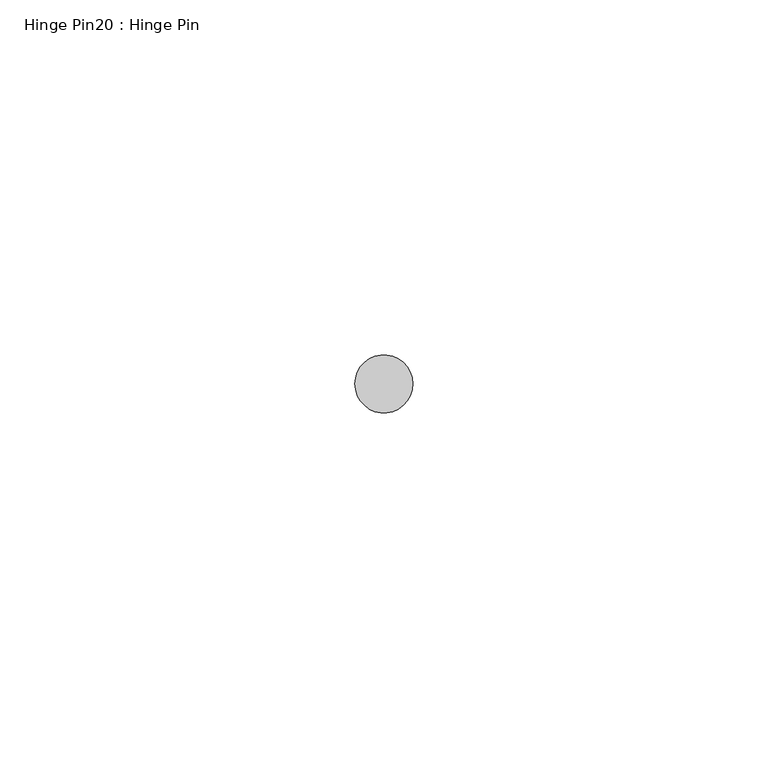
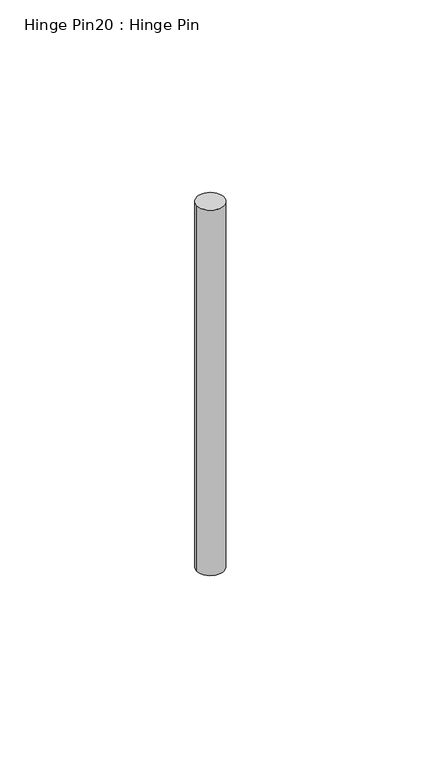
"""IFC4 building model written with IfcOpenShell, lengths in millimetres: proxy geometry, Hinge Pin20 : Hinge Pin."""

from ifc_helpers import new_model, si_unit, point, frame, frame_2d, origin, place, context, project, spatial, circle_curve, trimmed, segment, composite_curve, outline, extrude, source, transform, mapped, element, save


def hinge_pin20_hinge_pin_bc855f33(model_context):
    return source(origin(), model_context, "Body", "SweptSolid", [
        extrude(outline(composite_curve([segment(trimmed(circle_curve(frame_2d((587319.1320739, -534100.7049841)), 4.0894), [point((587315.0426739, -534100.7049841))], [point((587323.2214739, -534100.7049841))], False, "CARTESIAN"), True, "CONTINUOUS"), segment(trimmed(circle_curve(frame_2d((587319.1320739, -534100.7049841)), 4.0894), [point((587323.2214739, -534100.7049841))], [point((587315.0426739, -534100.7049841))], False, "CARTESIAN"), True, "CONTINUOUS")], self_intersect=False)), frame((0.0, 0.0, 1128.5140625), z_axis=(0.0, 0.0, 1.0), x_axis=(1.0, 0.0, 0.0)), (0.0, 0.0, 1.0), 117.871875),
    ])


if __name__ == "__main__":
    model = new_model("IFC4")
    model_context = context("Model", 3, world=origin())
    ifc_project = project(units=[si_unit("LENGTHUNIT", "METRE", prefix="MILLI")], contexts=[model_context])
    site = spatial("IfcSite", under=ifc_project)
    building = spatial("IfcBuilding", under=site)
    placement = place(None, origin())
    hinge_pin20_hinge_pin_shape = hinge_pin20_hinge_pin_bc855f33(model_context)
    element("IfcBuildingElementProxy", 1, Name="Hinge Pin20 : Hinge Pin", ObjectType="Hinge Pin20 : Hinge Pin", at=placement, inside=building, context=model_context, shape_type="MappedRepresentation", body=[
        mapped(hinge_pin20_hinge_pin_shape, transform((0.0, 0.0, 0.0), x_axis=(1.0, 0.0, 0.0), y_axis=(0.0, 1.0, 0.0), z_axis=(0.0, 0.0, 1.0))),
    ])
    save(model, "model.ifc")

# Revit data of these elements
# Element 1 (IfcBuildingElementProxy, "Hinge Pin20 : Hinge Pin")
#   Materials on its faces: "6\"X6\" WELD-ON STL BUTT HINGE"
# Materials
#   "6\"X6\" WELD-ON STL BUTT HINGE": class "Metal", colour RGB 189 187 185, transparency 0, Description = "Carbon steel", Cost = 0
